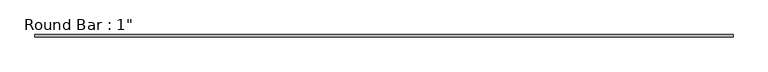
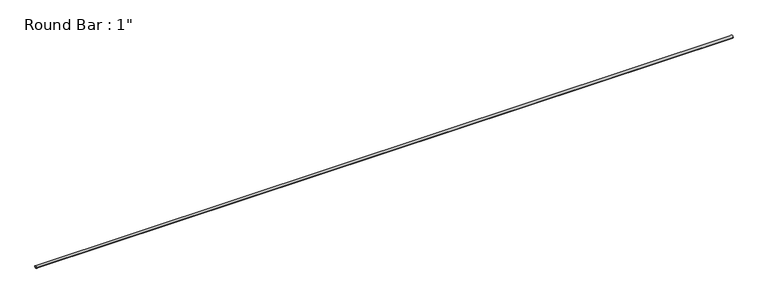
"""IFC4 building model written with IfcOpenShell, lengths in millimetres: member geometry."""

from ifc_helpers import new_model, si_unit, point, frame, origin, origin_2d, place, context, project, spatial, circle_curve, trimmed, segment, composite_curve, outline, extrude, source, transform, mapped, element, save


def member_3c518b88(model_context):
    return source(origin(), model_context, "Body", "SweptSolid", [
        extrude(outline(composite_curve([segment(trimmed(circle_curve(origin_2d(), 12.7), [point((-12.7, 0.0))], [point((12.7, 0.0))], False, "CARTESIAN"), True, "CONTINUOUS"), segment(trimmed(circle_curve(origin_2d(), 12.7), [point((12.7, 0.0))], [point((-12.7, 0.0))], False, "CARTESIAN"), True, "CONTINUOUS")], self_intersect=False)), frame((-3472.6994675, 0.0, 0.0), z_axis=(1.0, 0.0, 0.0), x_axis=(0.0, 1.0, 0.0)), (0.0, 0.0, 1.0), 6945.398935),
    ])


if __name__ == "__main__":
    model = new_model("IFC4")
    model_context = context("Model", 3, world=origin())
    ifc_project = project(units=[si_unit("LENGTHUNIT", "METRE", prefix="MILLI")], contexts=[model_context])
    site = spatial("IfcSite", under=ifc_project)
    building = spatial("IfcBuilding", under=site)
    placement = place(None, origin())
    member_shape = member_3c518b88(model_context)
    element("IfcMember", 1, ObjectType="Round Bar : 1\"", at=placement, inside=building, context=model_context, shape_type="MappedRepresentation", body=[
        mapped(member_shape, transform((0.0, 0.0, 0.0), x_axis=(1.0, 0.0, 0.0), y_axis=(0.0, 1.0, 0.0), z_axis=(0.0, 0.0, 1.0))),
    ])
    save(model, "model.ifc")

# Revit data of these elements
# Type "Round Bar : 1\""
#   Assembly Code = "B10"
#   W = 0
#   Start Extension Calculation [instance default] = 10' - 0"
#   Start Extension [instance default] = -0' - 0 1/2"
#   End Extension Calculation [instance default] = 10' - 0"
#   End Extension [instance default] = -0' - 0 1/2"
#   Length [instance default] = 5' - 0"
#   d = 0' - 1"
#   A = 0 SF
#   Structural Material [instance default] = Metal - Steel - ASTM A36
# Element 1 (IfcMember, "Round Bar : 1\"")
#   Materials on its faces: "Metal - Steel - ASTM A36"
# Materials
#   "Metal - Steel - ASTM A36": class "Metal", colour RGB 199 199 199, transparency 0
